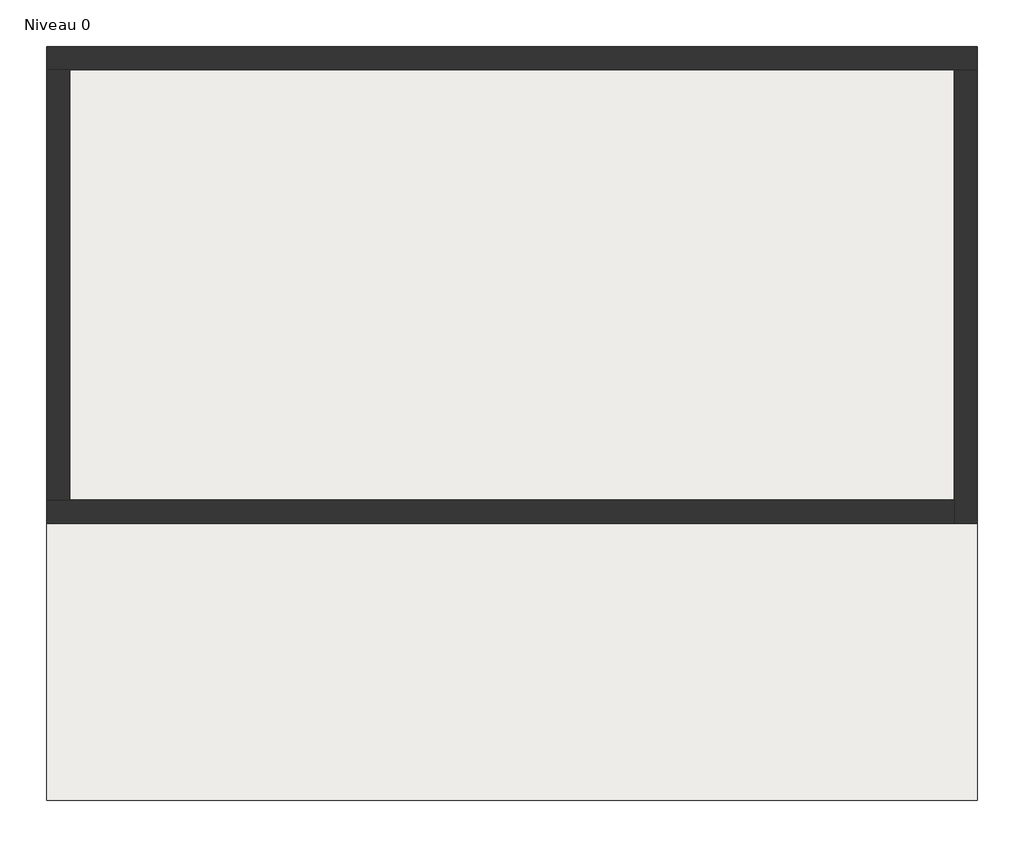
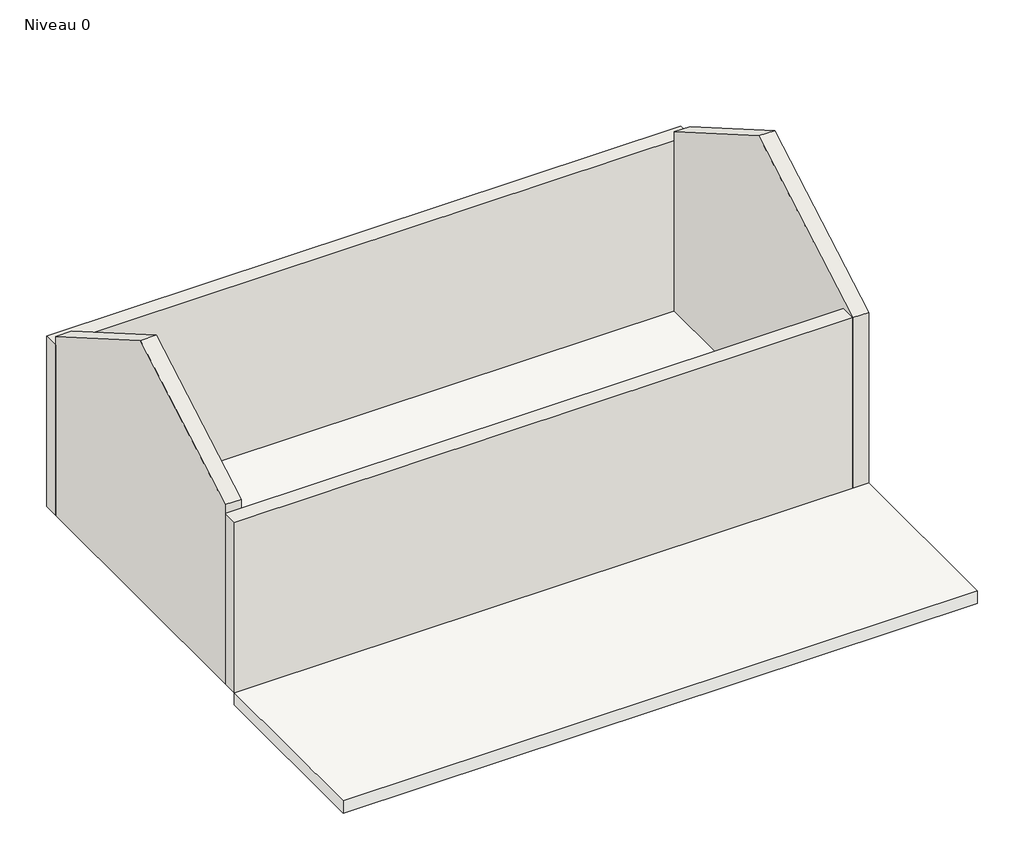
# One storey: 4 walls, 2 slabs.
"""IFC4 building model written with IfcOpenShell, lengths in millimetres."""

from ifc_helpers import new_model, si_unit, frame, origin, place, context, project, spatial, polyline, outline, extrude, faceted_brep, element, save

model = new_model("IFC4")

# Units and contexts
model_context = context("Model", 3, world=origin())
ifc_project = project(units=[si_unit("LENGTHUNIT", "METRE", prefix="MILLI")], contexts=[model_context])

# Site, building, storey
site = spatial("IfcSite", under=ifc_project)
building = spatial("IfcBuilding", under=site)
storey = spatial("IfcBuildingStorey", under=building, Name="Niveau 0", Elevation=0.0)

# Slabs
placement = place(None, origin())
element("IfcSlab", 1, ObjectType="Dalle en béton - 250 mm", at=placement, inside=storey, context=model_context, shape_type="SweptSolid", body=[
    extrude(outline(polyline([(2100.603041, 9444.9844082), (2100.603041, 3754.9844082), (-9589.396959, 3754.9844082), (-9589.396959, 9444.9844082), (2100.603041, 9444.9844082)])), frame((0.0, 0.0, -250.0), z_axis=(0.0, 0.0, 1.0), x_axis=(1.0, 0.0, 0.0)), (0.0, 0.0, 1.0), 250.0),
])
element("IfcSlab", 2, ObjectType="Dalle en béton - 250 mm", at=placement, inside=storey, context=model_context, shape_type="SweptSolid", body=[
    extrude(outline(polyline([(2410.603041, 3444.9844082), (2410.603041, -216.4554464), (-9899.396959, -216.4554464), (-9899.396959, 3444.9844082), (2410.603041, 3444.9844082)])), frame((0.0, 0.0, -250.0), z_axis=(0.0, 0.0, 1.0), x_axis=(1.0, 0.0, 0.0)), (0.0, 0.0, 1.0), 250.0),
])

# Walls
element("IfcWall", 3, ObjectType="mur 3", at=placement, inside=storey, context=model_context, shape_type="Brep", body=[
    faceted_brep([(-9899.396959, 9444.9844082, 0.0), (-9589.396959, 9444.9844082, 0.0), (2100.603041, 9444.9844082, 0.0), (2410.603041, 9444.9844082, 0.0), (2410.603041, 9444.9844082, 3500.0), (-9899.396959, 9444.9844082, 3500.0), (-9899.396959, 9754.9844082, 0.0), (-9899.396959, 9754.9844082, 3500.0), (2410.603041, 9754.9844082, 3500.0), (2410.603041, 9754.9844082, 0.0)], [[[0, 1, 2, 3, 4, 5]], [[6, 7, 8, 9]], [[3, 2, 1, 0, 6, 9]], [[5, 4, 8, 7]], [[4, 3, 9, 8]], [[0, 5, 7, 6]]]),
])
element("IfcWall", 4, ObjectType="mur 3", at=placement, inside=storey, context=model_context, shape_type="Brep", body=[
    faceted_brep([(2100.603041, 9444.9844082, 0.0), (2100.603041, 3754.9844082, 0.0), (2100.603041, 3444.9844082, 0.0), (2100.603041, 3444.9844082, 3500.0), (2100.603041, 6599.9844082, 5321.5400993), (2100.603041, 9444.9844082, 3678.9785834), (2410.603041, 9444.9844082, 0.0), (2410.603041, 9444.9844082, 3500.0), (2410.603041, 9444.9844082, 3678.9785834), (2410.603041, 6599.9844082, 5321.5400993), (2410.603041, 3444.9844082, 3500.0), (2410.603041, 3444.9844082, 0.0)], [[[0, 1, 2, 3, 4, 5]], [[6, 7, 8, 9, 10, 11]], [[2, 1, 0, 6, 11]], [[0, 5, 8, 7, 6]], [[3, 2, 11, 10]], [[5, 4, 9, 8]], [[4, 3, 10, 9]]]),
])
element("IfcWall", 5, ObjectType="mur 3", at=placement, inside=storey, context=model_context, shape_type="Brep", body=[
    faceted_brep([(2100.603041, 3754.9844082, 0.0), (-9589.396959, 3754.9844082, 0.0), (-9899.396959, 3754.9844082, 0.0), (-9899.396959, 3754.9844082, 3500.0), (2100.603041, 3754.9844082, 3500.0), (2100.603041, 3444.9844082, 0.0), (2100.603041, 3444.9844082, 3500.0), (-9899.396959, 3444.9844082, 3500.0), (-9899.396959, 3444.9844082, 0.0)], [[[0, 1, 2, 3, 4]], [[5, 6, 7, 8]], [[2, 1, 0, 5, 8]], [[4, 3, 7, 6]], [[0, 4, 6, 5]], [[3, 2, 8, 7]]]),
])
element("IfcWall", 6, ObjectType="mur 3", at=placement, inside=storey, context=model_context, shape_type="Brep", body=[
    faceted_brep([(-9589.396959, 3754.9844082, 0.0), (-9589.396959, 9444.9844082, 0.0), (-9589.396959, 9444.9844082, 3678.9785834), (-9589.396959, 6599.9844082, 5321.5400993), (-9589.396959, 3754.9844082, 3678.9785834), (-9899.396959, 3754.9844082, 0.0), (-9899.396959, 3754.9844082, 3500.0), (-9899.396959, 3754.9844082, 3678.9785834), (-9899.396959, 6599.9844082, 5321.5400993), (-9899.396959, 9444.9844082, 3678.9785834), (-9899.396959, 9444.9844082, 3500.0), (-9899.396959, 9444.9844082, 0.0)], [[[0, 1, 2, 3, 4]], [[5, 6, 7, 8, 9, 10, 11]], [[1, 0, 5, 11]], [[2, 1, 11, 10, 9]], [[0, 4, 7, 6, 5]], [[4, 3, 8, 7]], [[3, 2, 9, 8]]]),
])

save(model, "model.ifc")

# Revit data of these elements
# Project information
#   Date de fin du projet = "Date de fin"
#   Etat du projet = "Etat du projet"
#   Nom du client = "Propriétaire"
#   Adresse du projet = "Entrer l'adresse ici"
#   Nom du projet = "Nom du projet"
#   Numéro de projet = "0001"
# Type "Dalle en béton - 250 mm"
#   Function = 0
#   Layers, outside or top first: 0.25 m "Maçonnerie - Béton" (function 1)
# Type "mur 3"
#   Description = ""
#   Layers, outside or top first: 0.20 m "Mur par défaut" (function 1); 0.10 m no material (function 3); 0.01 m no material (function 4)
# Elements 1, 2 (IfcSlab, "Dalle en béton - 250 mm")
#   Height Offset From Level = 0.00 m
#   Phase Created = Nouvelle construction
#   Materials on its faces: "Maçonnerie - Béton"
# Elements 3, 4, 5, 6 (IfcWall, "mur 3")
#   Top Offset = 0.00 m
#   Base Offset = 0.00 m
#   wall height = 3.50 m
#   Phase Created = Nouvelle construction
#   Base Constraint = Niveau 0
#   Top Constraint = Niveau 1
#   Materials on its faces: "Mur par défaut"
# Materials
#   "Maçonnerie - Béton": class "Béton", colour RGB 153 162 160, transparency 0, Cost = 0
#   "Mur par défaut": class "Divers", colour RGB 142 140 122, transparency 0, Cost = 0
